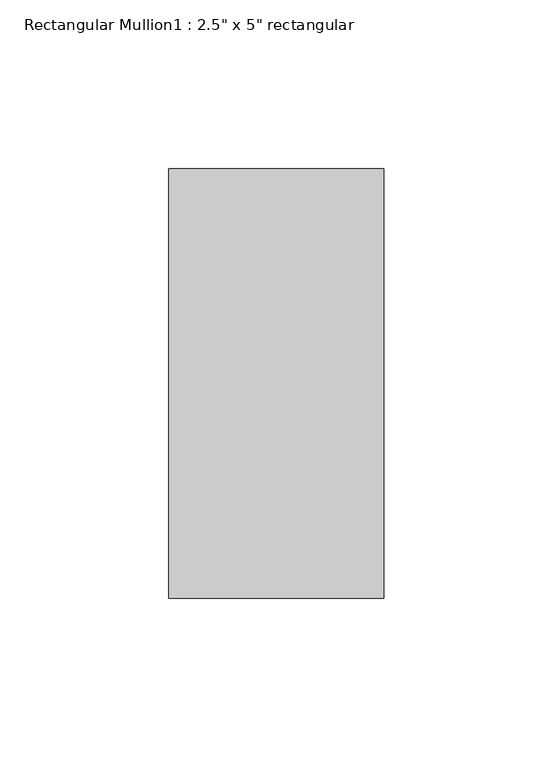
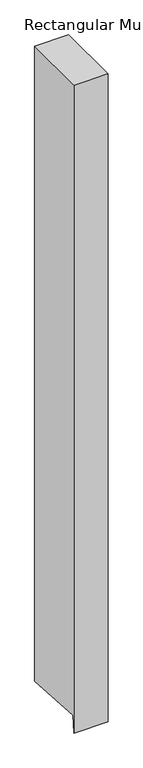
"""IFC4 building model written with IfcOpenShell, lengths in millimetres: member geometry."""

from ifc_helpers import new_model, si_unit, frame, origin, place, context, project, spatial, polyline, outline, extrude, source, transform, mapped, element, save


def member_2ae322fc(model_context):
    return source(origin(), model_context, "Body", "SweptSolid", [
        extrude(outline(polyline([(-63.5, 0.0), (63.5, 0.0), (63.5, -1253.5867756), (-61.1522336, -1244.9455147), (-63.5, -1278.8126009), (-63.5, 0.0)])), frame((-63.5, 0.0, 0.0), z_axis=(1.0, 0.0, 0.0), x_axis=(0.0, 1.0, 0.0)), (0.0, 0.0, 1.0), 63.5),
    ])


if __name__ == "__main__":
    model = new_model("IFC4")
    model_context = context("Model", 3, world=origin())
    ifc_project = project(units=[si_unit("LENGTHUNIT", "METRE", prefix="MILLI")], contexts=[model_context])
    site = spatial("IfcSite", under=ifc_project)
    building = spatial("IfcBuilding", under=site)
    placement = place(None, origin())
    member_shape = member_2ae322fc(model_context)
    element("IfcMember", 1, ObjectType="Rectangular Mullion1 : 2.5\" x 5\" rectangular", at=placement, inside=building, context=model_context, shape_type="MappedRepresentation", body=[
        mapped(member_shape, transform((0.0, 0.0, 0.0), x_axis=(1.0, 0.0, 0.0), y_axis=(0.0, 1.0, 0.0), z_axis=(0.0, 0.0, 1.0))),
    ])
    save(model, "model.ifc")

# Revit data of these elements
# Type "Rectangular Mullion1 : 2.5\" x 5\" rectangular"
#   built-in parameter 1007304 = 0.416667 (stored number, unit not read)
#   built-in parameter 1007301 = 0.104167 (stored number, unit not read)
#   built-in parameter 1007300 = 0.104167 (stored number, unit not read)
# Element 1 (IfcMember, "Rectangular Mullion1 : 2.5\" x 5\" rectangular")
#   Materials on its faces: "support-frame"
# Materials
#   "support-frame": class "Unassigned", colour RGB 233 233 233, transparency 0, Cost = 0
